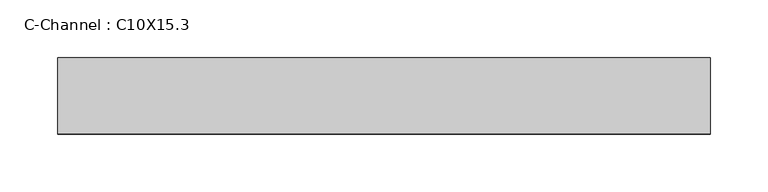
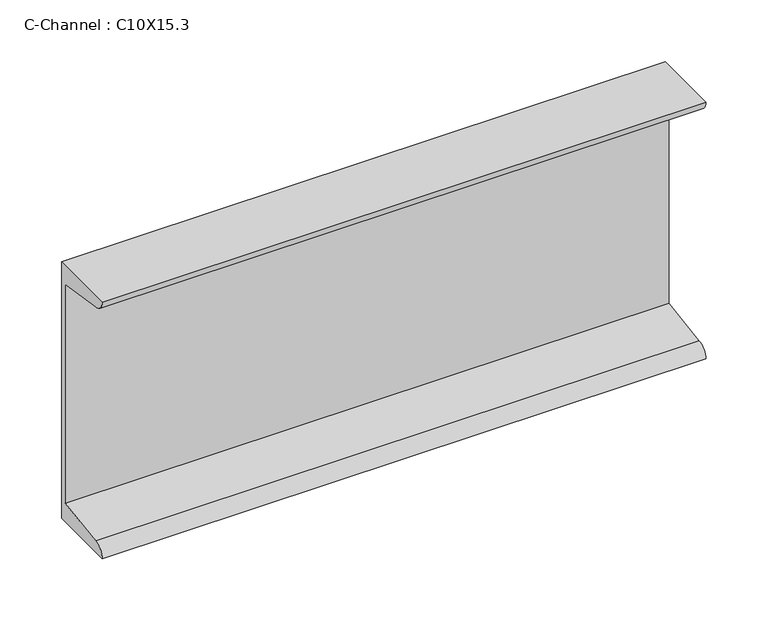
"""IFC4 building model written with IfcOpenShell, lengths in millimetres: beam geometry, C-Channel : C10X15.3."""

from ifc_helpers import new_model, si_unit, point, frame, frame_2d, origin, place, context, project, spatial, polyline, circle_curve, trimmed, segment, composite_curve, outline, extrude, source, transform, mapped, element, save


def c_channel_c10x15_3_a7bd5103(model_context):
    return source(origin(), model_context, "Body", "SweptSolid", [
        extrude(outline(composite_curve([segment(polyline([(16.1036, 127.0), (16.1036, -127.0), (-49.9364, -127.0)]), True, "CONTINUOUS"), segment(trimmed(circle_curve(frame_2d((-38.862, -127.0)), 11.0744), [point((-49.9364, -127.0))], [point((-38.862, -115.9256))], False, "CARTESIAN"), True, "CONTINUOUS"), segment(polyline([(-38.862, -115.9256), (10.0076, -108.1854158), (10.0076, 108.1854158), (-38.862, 115.9256)]), True, "CONTINUOUS"), segment(trimmed(circle_curve(frame_2d((-38.862, 127.0)), 11.0744), [point((-38.862, 115.9256))], [point((-49.9364, 127.0))], False, "CARTESIAN"), True, "CONTINUOUS"), segment(polyline([(-49.9364, 127.0), (16.1036, 127.0)]), True, "CONTINUOUS")], self_intersect=False)), frame((-292.1, 0.0, 0.0), z_axis=(1.0, 0.0, 0.0), x_axis=(0.0, 1.0, 0.0)), (0.0, 0.0, 1.0), 565.15),
    ])


if __name__ == "__main__":
    model = new_model("IFC4")
    model_context = context("Model", 3, world=origin())
    ifc_project = project(units=[si_unit("LENGTHUNIT", "METRE", prefix="MILLI")], contexts=[model_context])
    site = spatial("IfcSite", under=ifc_project)
    building = spatial("IfcBuilding", under=site)
    placement = place(None, origin())
    c_channel_c10x15_3_shape = c_channel_c10x15_3_a7bd5103(model_context)
    element("IfcBeam", 1, ObjectType="C-Channel : C10X15.3", at=placement, inside=building, context=model_context, shape_type="MappedRepresentation", body=[
        mapped(c_channel_c10x15_3_shape, transform((0.0, 0.0, 0.0), x_axis=(1.0, 0.0, 0.0), y_axis=(0.0, 1.0, 0.0), z_axis=(0.0, 0.0, 1.0))),
    ])
    save(model, "model.ifc")

# Revit data of these elements
# Type "C-Channel : C10X15.3"
#   Assembly Code = "B10"
#   W = 15.3
#   Length [instance default] = 5' - 0"
#   bf = 0' - 2.6"
#   d = 0' - 10"
#   tf = 0' - 0.436"
#   tw = 0' - 0.24"
#   x = 0' - 0.634"
#   A = 0.0311111 SF
#   Structural Material [instance default] = Steel ASTM A36
# Element 1 (IfcBeam, "C-Channel : C10X15.3")
#   Structural Material = Steel ASTM A992
#   Materials on its faces: "Steel ASTM A992"
# Materials
#   "Steel ASTM A36": class "Metal", colour RGB 199 199 199, transparency 0, Description = "Structural steel, ASTM A36 Grade B, mill finish", Cost = 0
#   "Steel ASTM A992": class "Metal", colour RGB 199 199 199, transparency 0, Description = "Structural steel 50ksi", Cost = 0
